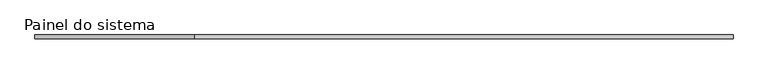
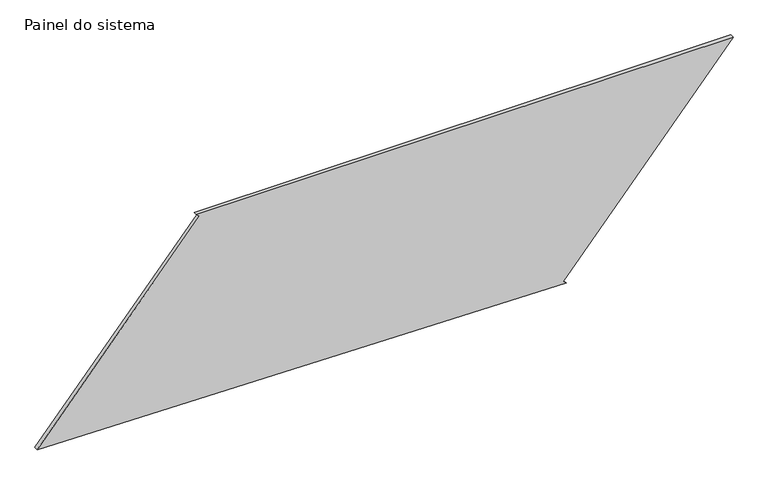
"""IFC4 building model written with IfcOpenShell, lengths in millimetres: plate geometry, Painel do sistema : Envidraçado."""

from ifc_helpers import new_model, si_unit, frame, origin, place, context, project, spatial, polyline, outline, extrude, source, transform, mapped, element, save


def painel_do_sistema_6114ac98(model_context):
    return source(origin(), model_context, "Body", "SweptSolid", [
        extrude(outline(polyline([(0.0, 1129.8098197), (16.2242617, 1110.7894798), (1259.1222132, 2170.9756657), (1259.1222132, -1177.5829638), (1242.8979515, -1158.5626238), (56.0063352, -2170.9756657), (0.0, 1129.8098197)])), frame((0.0, 24.5, 0.0), z_axis=(0.0, 1.0, 0.0), x_axis=(0.0, 0.0, 1.0)), (0.0, 0.0, 1.0), 25.0),
    ])


if __name__ == "__main__":
    model = new_model("IFC4")
    model_context = context("Model", 3, world=origin())
    ifc_project = project(units=[si_unit("LENGTHUNIT", "METRE", prefix="MILLI")], contexts=[model_context])
    site = spatial("IfcSite", under=ifc_project)
    building = spatial("IfcBuilding", under=site)
    placement = place(None, origin())
    painel_do_sistema_shape = painel_do_sistema_6114ac98(model_context)
    element("IfcPlate", 1, ObjectType="Painel do sistema : Envidraçado", at=placement, inside=building, context=model_context, shape_type="MappedRepresentation", body=[
        mapped(painel_do_sistema_shape, transform((0.0, 0.0, 0.0), x_axis=(1.0, 0.0, 0.0), y_axis=(0.0, 1.0, 0.0), z_axis=(0.0, 0.0, 1.0))),
    ])
    save(model, "model.ifc")

# Revit data of these elements
# Type "Painel do sistema : Envidraçado"
#   Construction Type Id = "GSP4R"
#   Analytic Construction = "Vidraça única Pilkington 1/8 pol"
#   Visual Light Transmittance = 0.9
#   Solar Heat Gain Coefficient = 0.86
#   Heat Transfer Coefficient (U) = 6.7069 W/(m²·K)
# Element 1 (IfcPlate, "Painel do sistema : Envidraçado")
#   Materials on its faces: "Vidro"
# Materials
#   "Vidro": class "Vidro", colour RGB 0 128 192, transparency 0.9, Description = "Vidro de sílica", Cost = 0
